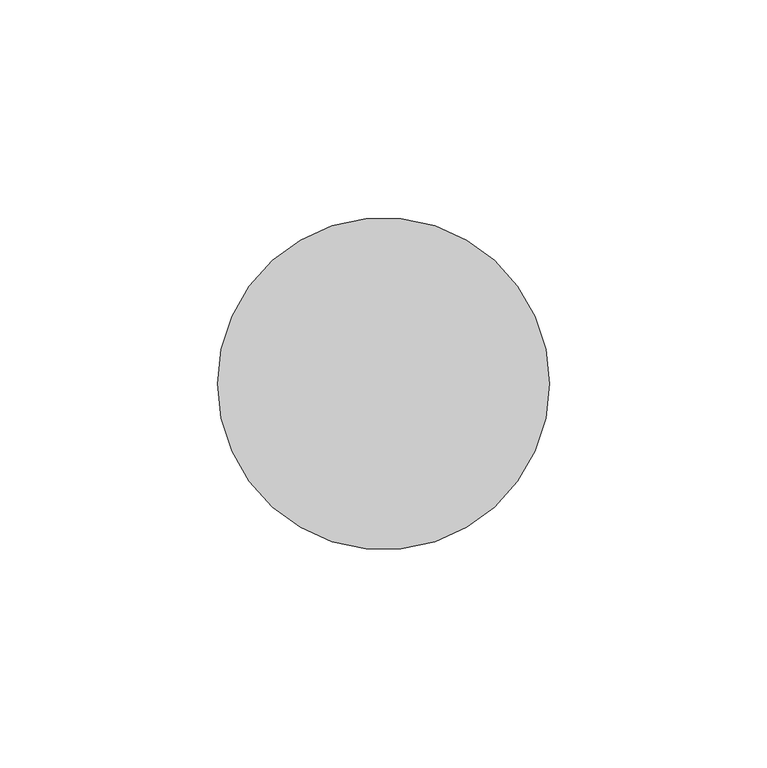
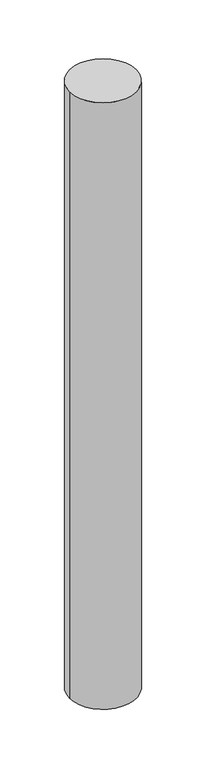
"""IFC4 building model written with IfcOpenShell, lengths in millimetres: furniture geometry, Kietchen Desk Leg : Kietchen Desk Leg."""

from ifc_helpers import new_model, si_unit, point, frame, origin, place, context, project, spatial, circle_curve, ellipse_curve, trimmed, source, transform, mapped, element, save
from ifc_brep_helpers import plane_surface, extruded_surface, advanced_brep


def furniture_ec399a33(model_context):
    return source(origin(), model_context, "Body", "AdvancedBrep", [
        advanced_brep(
        [(4373.1537589, 8746.4712165, 732.3567917), (4296.9537589, 8746.4712165, 732.3567917), (4373.1537589, 8746.4712165, 0.0), (4296.9537589, 8746.4712165, 0.0)],
        [
            (0, 1, circle_curve(frame((4335.0537589, 8746.4712165, 732.3567917), z_axis=(0.0, 0.0, 1.0), x_axis=(-1.0, 0.0, 0.0)), 38.1)),
            (1, 0, circle_curve(frame((4335.0537589, 8746.4712165, 732.3567917), z_axis=(0.0, 0.0, 1.0), x_axis=(-1.0, 0.0, 0.0)), 38.1)),
            (2, 3, ellipse_curve(frame((4335.0537589, 8746.4712165, 0.0), z_axis=(0.0, 0.0, -1.0), x_axis=(-1.0, 0.0, 0.0)), 38.1, 38.1)),
            (3, 2, ellipse_curve(frame((4335.0537589, 8746.4712165, 0.0), z_axis=(0.0, 0.0, -1.0), x_axis=(-1.0, 0.0, 0.0)), 38.1, 38.1)),
            (0, 2),
            (3, 1),
        ],
        [
            plane_surface(frame((4296.9537589, 8746.4712165, 732.3567917), z_axis=(0.0, 0.0, 1.0), x_axis=(0.0, -1.0, 0.0))),
            plane_surface(frame((4296.9537589, 8746.4712165, 0.0), z_axis=(0.0, 0.0, -1.0), x_axis=(0.0, 1.0, 0.0))),
            extruded_surface(trimmed(ellipse_curve(frame((4335.0537589, 8746.4712165, -732.3567917), z_axis=(0.0, 0.0, 1.0), x_axis=(-1.0, 0.0, 0.0)), 38.1, 38.1), [point((4373.1537589, 8746.4712165, -732.3567917))], [point((4296.9537589, 8746.4712165, -732.3567917))], True, "CARTESIAN"), (0.0, 0.0, 732.3567917), 732.3567917),
            extruded_surface(trimmed(ellipse_curve(frame((4335.0537589, 8746.4712165, -732.3567917), z_axis=(0.0, 0.0, 1.0), x_axis=(-1.0, 0.0, 0.0)), 38.1, 38.1), [point((4296.9537589, 8746.4712165, -732.3567917))], [point((4373.1537589, 8746.4712165, -732.3567917))], True, "CARTESIAN"), (0.0, 0.0, 732.3567917), 732.3567917),
        ],
        [
            (0, [[1, 2]]),
            (1, [[3, 4]]),
            (2, [[-1, 5, -4, 6]]),
            (3, [[-2, -6, -3, -5]]),
        ],
    ),
    ])


if __name__ == "__main__":
    model = new_model("IFC4")
    model_context = context("Model", 3, world=origin())
    ifc_project = project(units=[si_unit("LENGTHUNIT", "METRE", prefix="MILLI")], contexts=[model_context])
    site = spatial("IfcSite", under=ifc_project)
    building = spatial("IfcBuilding", under=site)
    placement = place(None, origin())
    furniture_shape = furniture_ec399a33(model_context)
    element("IfcFurniture", 1, ObjectType="Kietchen Desk Leg : Kietchen Desk Leg", at=placement, inside=building, context=model_context, shape_type="MappedRepresentation", body=[
        mapped(furniture_shape, transform((0.0, 0.0, 0.0), x_axis=(1.0, 0.0, 0.0), y_axis=(0.0, 1.0, 0.0), z_axis=(0.0, 0.0, 1.0))),
    ])
    save(model, "model.ifc")

# Revit data of these elements
# Type "Kietchen Desk Leg : Kietchen Desk Leg"
#   COBie.Type = no
# Element 1 (IfcFurniture, "Kietchen Desk Leg : Kietchen Desk Leg")
#   Materials on its faces: "Trim - White"
# Materials
#   "Trim - White": class "Wood", colour RGB 255 255 255, transparency 0, Cost = 0
